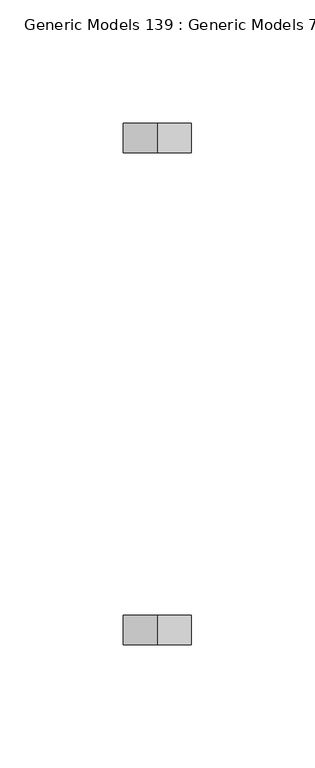
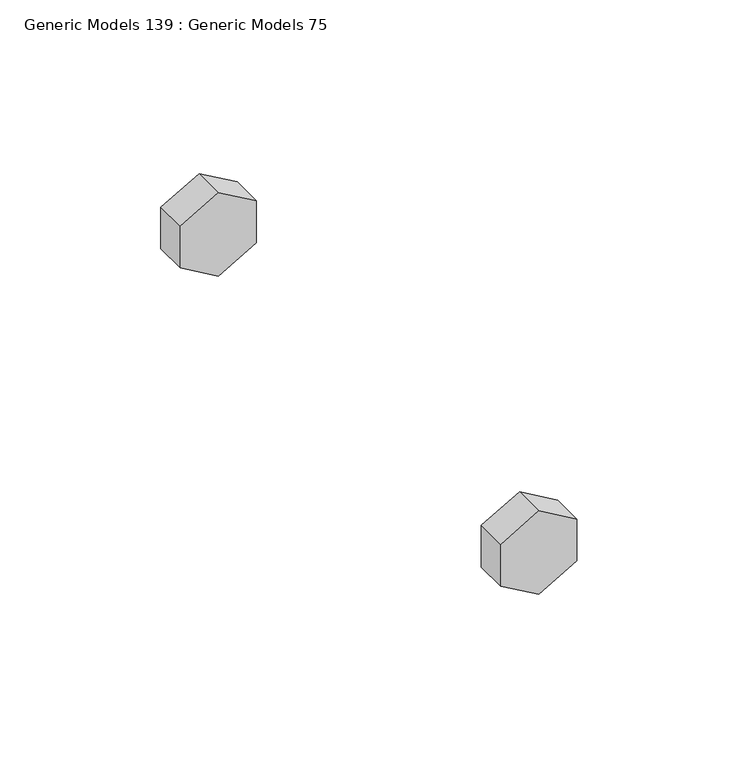
"""IFC4 building model written with IfcOpenShell, lengths in millimetres: proxy geometry, Generic Models 139 : Generic Models 75."""

from ifc_helpers import new_model, si_unit, frame, origin, place, context, project, spatial, polyline, outline, extrude, source, transform, mapped, element, save


def generic_models_139_generic_models_75_0e24d838(model_context):
    return source(origin(), model_context, "Body", "SweptSolid", [
        extrude(outline(polyline([(268917.5462802, 31975.9942029), (268901.7097067, 31975.9942029), (268893.79142, 31989.7090778), (268901.7097067, 32003.4239528), (268917.5462802, 32003.4239528), (268925.464567, 31989.7090778), (268917.5462802, 31975.9942029)])), frame((0.0, 30868.0031612, 0.0), z_axis=(0.0, 1.0, 0.0), x_axis=(0.0, 0.0, 1.0)), (0.0, 0.0, 1.0), 11.90625),
        extrude(outline(polyline([(268917.5462802, 31975.9942029), (268901.7097067, 31975.9942029), (268893.79142, 31989.7090778), (268901.7097067, 32003.4239528), (268917.5462802, 32003.4239528), (268925.464567, 31989.7090778), (268917.5462802, 31975.9942029)])), frame((0.0, 30668.7719112, 0.0), z_axis=(0.0, 1.0, 0.0), x_axis=(0.0, 0.0, 1.0)), (0.0, 0.0, 1.0), 11.90625),
    ])


if __name__ == "__main__":
    model = new_model("IFC4")
    model_context = context("Model", 3, world=origin())
    ifc_project = project(units=[si_unit("LENGTHUNIT", "METRE", prefix="MILLI")], contexts=[model_context])
    site = spatial("IfcSite", under=ifc_project)
    building = spatial("IfcBuilding", under=site)
    placement = place(None, origin())
    generic_models_139_generic_models_75_shape = generic_models_139_generic_models_75_0e24d838(model_context)
    element("IfcBuildingElementProxy", 1, Name="Generic Models 139 : Generic Models 75", ObjectType="Generic Models 139 : Generic Models 75", at=placement, inside=building, context=model_context, shape_type="MappedRepresentation", body=[
        mapped(generic_models_139_generic_models_75_shape, transform((0.0, 0.0, 0.0), x_axis=(1.0, 0.0, 0.0), y_axis=(0.0, 1.0, 0.0), z_axis=(0.0, 0.0, 1.0))),
    ])
    save(model, "model.ifc")

# Revit data of these elements
# Element 1 (IfcBuildingElementProxy, "Generic Models 139 : Generic Models 75")
#   Materials on its faces: "3/4\" GALV. THRU BOLTS"
# Materials
#   "3/4\" GALV. THRU BOLTS": class "Generic", colour RGB 105 69 171, transparency 0, Cost = 0
